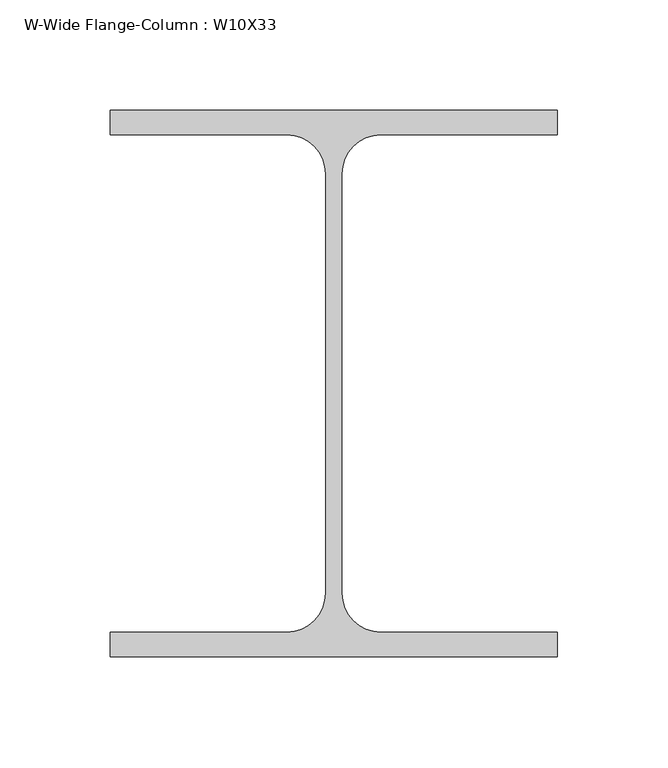
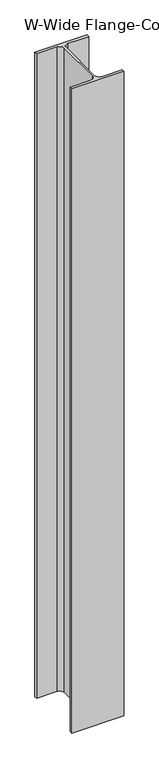
"""IFC4 building model written with IfcOpenShell, lengths in millimetres: column geometry, W-Wide Flange-Column : W10X33."""

import ifcopenshell
import ifcopenshell.guid

model = None  # the IFC model being written
_history = None  # IfcOwnerHistory: only IFC2X3 demands one
_inside = {}  # id of a spatial element -> (the spatial element, [elements in it])
_under = {}  # id of a project, library or spatial element -> (it, [spatial elements below it])
_declared = {}  # id of a project -> (the project, [libraries it declares])
_typed = {}  # id of a type object -> (the type object, [elements of that type])
_made_of = {}  # id of a material, layer set ... -> (it, [elements and type objects made of it])


def new_model(schema):
    """Start an empty IFC model of exactly this schema.

    Asked for "IFC4X3", IfcOpenShell would pick the latest addendum, in which some entities
    have other attributes; the version numbers below select the first issue.
    IFC2X3 requires an IfcOwnerHistory on every rooted entity: one is made here for all.
    """
    global model, _history
    if schema == "IFC4X3":
        model = ifcopenshell.file(schema_version=(4, 3, 0, 0))
    else:
        model = ifcopenshell.file(schema=schema)
    _inside.clear()
    _under.clear()
    _declared.clear()
    _typed.clear()
    _made_of.clear()
    _history = None
    if model.schema == "IFC2X3":
        org = make("IfcOrganization", Name="unknown")
        user = make(
            "IfcPersonAndOrganization",
            ThePerson=make("IfcPerson", FamilyName="unknown"),
            TheOrganization=org,
        )
        app = make(
            "IfcApplication",
            ApplicationDeveloper=org,
            Version="unknown",
            ApplicationFullName="unknown",
            ApplicationIdentifier="unknown",
        )
        _history = make(
            "IfcOwnerHistory",
            OwningUser=user,
            OwningApplication=app,
            ChangeAction="ADDED",
            CreationDate=0,
        )
    return model


def make(cls, **values):
    """One entity of the class cls with the attributes given. An attribute that is None is left unset."""
    return model.create_entity(
        cls, **{name: value for name, value in values.items() if value is not None}
    )


def rooted(cls, **values):
    """An entity with a GlobalId (a new one), such as an element, a storey or a relation."""
    return make(cls, GlobalId=ifcopenshell.guid.new(), OwnerHistory=_history, **values)


def si_unit(unit_type, name, prefix=None):
    """IfcSIUnit, for example si_unit("LENGTHUNIT", "METRE", prefix="MILLI")."""
    return make("IfcSIUnit", UnitType=unit_type, Prefix=prefix, Name=name)


def assignment(units):
    """IfcUnitAssignment: the units of a project."""
    return None if units is None else make("IfcUnitAssignment", Units=units)


def point(xyz):
    """IfcCartesianPoint."""
    return None if xyz is None else make("IfcCartesianPoint", Coordinates=xyz)


def direction(xyz):
    """IfcDirection."""
    return None if xyz is None else make("IfcDirection", DirectionRatios=xyz)


def frame(location, z_axis=None, x_axis=None):
    """IfcAxis2Placement3D, a coordinate frame: its origin and axes. An axis left out is left unset."""
    return make(
        "IfcAxis2Placement3D",
        Location=point(location),
        Axis=direction(z_axis),
        RefDirection=direction(x_axis),
    )


def frame_2d(location, x_axis=None):
    """IfcAxis2Placement2D, a coordinate frame in the plane: its origin and x axis."""
    return make(
        "IfcAxis2Placement2D", Location=point(location), RefDirection=direction(x_axis)
    )


def origin():
    """The frame at (0, 0, 0) with its axes left unset."""
    return frame((0.0, 0.0, 0.0))


def place(relative_to, where):
    """IfcLocalPlacement: puts the frame where relative to a parent placement (None: the world)."""
    return make(
        "IfcLocalPlacement", PlacementRelTo=relative_to, RelativePlacement=where
    )


def context(
    kind, dimensions, precision=None, world=None, true_north=None, identifier=None
):
    """IfcGeometricRepresentationContext, for example the 3D "Model" context."""
    return make(
        "IfcGeometricRepresentationContext",
        ContextIdentifier=identifier,
        ContextType=kind,
        CoordinateSpaceDimension=dimensions,
        Precision=precision,
        WorldCoordinateSystem=world,
        TrueNorth=true_north,
    )


def project(units=None, contexts=None):
    """IfcProject with its units and contexts."""
    return rooted(
        "IfcProject",
        Name="project",
        RepresentationContexts=contexts,
        UnitsInContext=assignment(units),
    )


def spatial(cls, under=None, at=None, **own):
    """A site, building, storey or space (cls), placed at a placement, below another one or the project."""
    s = rooted(cls, ObjectPlacement=at, **own)
    if under is not None:
        _under.setdefault(under.id(), (under, []))[1].append(s)
    return s


def polyline(points):
    """IfcPolyline through the points."""
    return make("IfcPolyline", Points=[point(p) for p in points])


def circle_curve(where, radius):
    """IfcCircle in the frame where."""
    return make("IfcCircle", Position=where, Radius=radius)


def trimmed(basis, trim1, trim2, sense, master):
    """IfcTrimmedCurve: the piece of a basis curve between two trims."""
    return make(
        "IfcTrimmedCurve",
        BasisCurve=basis,
        Trim1=trim1,
        Trim2=trim2,
        SenseAgreement=sense,
        MasterRepresentation=master,
    )


def segment(curve, same_sense, transition):
    """IfcCompositeCurveSegment."""
    return make(
        "IfcCompositeCurveSegment",
        Transition=transition,
        SameSense=same_sense,
        ParentCurve=curve,
    )


def composite_curve(segments, self_intersect=None):
    """IfcCompositeCurve: segments joined end to end."""
    return make("IfcCompositeCurve", Segments=segments, SelfIntersect=self_intersect)


def outline(outer, holes=None, kind="AREA"):
    """IfcArbitraryClosedProfileDef: a profile drawn as a closed curve; with holes, ...WithVoids."""
    if holes is None:
        return make("IfcArbitraryClosedProfileDef", ProfileType=kind, OuterCurve=outer)
    return make(
        "IfcArbitraryProfileDefWithVoids",
        ProfileType=kind,
        OuterCurve=outer,
        InnerCurves=holes,
    )


def extrude(swept, where, along, depth):
    """IfcExtrudedAreaSolid: the profile swept, set in the frame where, extruded along a direction by depth."""
    return make(
        "IfcExtrudedAreaSolid",
        SweptArea=swept,
        Position=where,
        ExtrudedDirection=direction(along),
        Depth=depth,
    )


def shape(context_of_items, identifier, shape_type, items):
    """IfcShapeRepresentation: the items that make up one representation, for example the "Body"."""
    return make(
        "IfcShapeRepresentation",
        ContextOfItems=context_of_items,
        RepresentationIdentifier=identifier,
        RepresentationType=shape_type,
        Items=items,
    )


def source(mapping_origin, context_of_items, identifier, shape_type, items):
    """IfcRepresentationMap: a shape defined once, which mapped items show again and again."""
    return make(
        "IfcRepresentationMap",
        MappingOrigin=mapping_origin,
        MappedRepresentation=shape(context_of_items, identifier, shape_type, items),
    )


def transform(
    local_origin,
    x_axis=None,
    y_axis=None,
    z_axis=None,
    scale=None,
    scale2=None,
    scale3=None,
    uniform=True,
):
    """IfcCartesianTransformationOperator3D, or its non-uniform kind. x_axis, y_axis, z_axis: its Axis1, 2, 3."""
    if uniform:
        return make(
            "IfcCartesianTransformationOperator3D",
            Axis1=direction(x_axis),
            Axis2=direction(y_axis),
            LocalOrigin=point(local_origin),
            Scale=scale,
            Axis3=direction(z_axis),
        )
    return make(
        "IfcCartesianTransformationOperator3DnonUniform",
        Axis1=direction(x_axis),
        Axis2=direction(y_axis),
        LocalOrigin=point(local_origin),
        Scale=scale,
        Axis3=direction(z_axis),
        Scale2=scale2,
        Scale3=scale3,
    )


def mapped(mapping_source, mapping_target):
    """IfcMappedItem: shows the shape of a source again, moved by a transform."""
    return make(
        "IfcMappedItem", MappingSource=mapping_source, MappingTarget=mapping_target
    )


def made_of(thing, what):
    """Note that an element or type object is made of a material, layer set ...; save() writes the relation."""
    if what is not None:
        _made_of.setdefault(what.id(), (what, []))[1].append(thing)
    return thing


def element(
    cls,
    number,
    at=None,
    inside=None,
    cuts=None,
    type_object=None,
    material=None,
    context=None,
    identifier="Body",
    shape_type=None,
    held_by="IfcProductDefinitionShape",
    body=None,
    shapes=None,
    **own,
):
    """One element of the class cls, such as IfcWall. Its Tag is "e" and its number.

    at: its placement. inside: the storey or other place that contains it. cuts: it is an
    opening in that element (IfcRelVoidsElement). A single representation is given by context,
    identifier, shape_type and body (its items); several are given by shapes. held_by: the class
    of the entity that holds the representations. save() writes the other relations.
    """
    e = rooted(cls, Tag="e%d" % number, ObjectPlacement=at, **own)
    if body is not None:
        shapes = [shape(context, identifier, shape_type, body)]
    if shapes is not None:
        e.Representation = make(held_by, Representations=shapes)
    if inside is not None:
        _inside.setdefault(inside.id(), (inside, []))[1].append(e)
    if cuts is not None:
        rooted(
            "IfcRelVoidsElement", RelatingBuildingElement=cuts, RelatedOpeningElement=e
        )
    if type_object is not None:
        _typed.setdefault(type_object.id(), (type_object, []))[1].append(e)
    return made_of(e, material)


def aggregate(whole, parts):
    """IfcRelAggregates: a whole, such as a stair, and the parts it consists of."""
    return rooted("IfcRelAggregates", RelatingObject=whole, RelatedObjects=parts)


def save(model, path):
    """Write the relations noted so far, then the file.

    IfcRelAggregates (storeys below a building ...), IfcRelContainedInSpatialStructure (elements
    in a storey), IfcRelDefinesByType, IfcRelAssociatesMaterial and IfcRelDeclares: one each for
    every whole, place, type object, material and project.
    """
    for whole, parts in _under.values():
        aggregate(whole, parts)
    for where, things in _inside.values():
        rooted(
            "IfcRelContainedInSpatialStructure",
            RelatedElements=things,
            RelatingStructure=where,
        )
    for kind, things in _typed.values():
        rooted("IfcRelDefinesByType", RelatedObjects=things, RelatingType=kind)
    for what, things in _made_of.values():
        rooted("IfcRelAssociatesMaterial", RelatedObjects=things, RelatingMaterial=what)
    for by, libraries in _declared.values():
        rooted("IfcRelDeclares", RelatingContext=by, RelatedDefinitions=libraries)
    model.write(path)


def w_wide_flange_column_w10x33_651e5602(model_context):
    return source(origin(), model_context, "Body", "SweptSolid", [
        extrude(outline(composite_curve([segment(polyline([(101.092, 123.571), (101.092, 112.522), (21.209, 112.522)]), True, "CONTINUOUS"), segment(trimmed(circle_curve(frame_2d((21.209, 94.996)), 17.526), [point((21.209, 112.522))], [point((3.683, 94.996))], True, "CARTESIAN"), True, "CONTINUOUS"), segment(polyline([(3.683, 94.996), (3.683, -94.996)]), True, "CONTINUOUS"), segment(trimmed(circle_curve(frame_2d((21.209, -94.996)), 17.526), [point((3.683, -94.996))], [point((21.209, -112.522))], True, "CARTESIAN"), True, "CONTINUOUS"), segment(polyline([(21.209, -112.522), (101.092, -112.522), (101.092, -123.571), (-101.092, -123.571), (-101.092, -112.522), (-21.209, -112.522)]), True, "CONTINUOUS"), segment(trimmed(circle_curve(frame_2d((-21.209, -94.996)), 17.526), [point((-21.209, -112.522))], [point((-3.683, -94.996))], True, "CARTESIAN"), True, "CONTINUOUS"), segment(polyline([(-3.683, -94.996), (-3.683, 94.996)]), True, "CONTINUOUS"), segment(trimmed(circle_curve(frame_2d((-21.209, 94.996)), 17.526), [point((-3.683, 94.996))], [point((-21.209, 112.522))], True, "CARTESIAN"), True, "CONTINUOUS"), segment(polyline([(-21.209, 112.522), (-101.092, 112.522), (-101.092, 123.571), (101.092, 123.571)]), True, "CONTINUOUS")], self_intersect=False)), frame((0.0, 0.0, 19253.2), z_axis=(0.0, 0.0, 1.0), x_axis=(1.0, 0.0, 0.0)), (0.0, 0.0, 1.0), 2641.6),
    ])


if __name__ == "__main__":
    model = new_model("IFC4")
    model_context = context("Model", 3, world=origin())
    ifc_project = project(units=[si_unit("LENGTHUNIT", "METRE", prefix="MILLI")], contexts=[model_context])
    site = spatial("IfcSite", under=ifc_project)
    building = spatial("IfcBuilding", under=site)
    placement = place(None, origin())
    w_wide_flange_column_w10x33_shape = w_wide_flange_column_w10x33_651e5602(model_context)
    element("IfcColumn", 1, ObjectType="W-Wide Flange-Column : W10X33", at=placement, inside=building, context=model_context, shape_type="MappedRepresentation", body=[
        mapped(w_wide_flange_column_w10x33_shape, transform((0.0, 0.0, 0.0), x_axis=(1.0, 0.0, 0.0), y_axis=(0.0, 1.0, 0.0), z_axis=(0.0, 0.0, 1.0))),
    ])
    save(model, "model.ifc")

# Revit data of these elements
# Type "W-Wide Flange-Column : W10X33"
#   Assembly Code = "B10"
#   W = 33
#   bf = 0' - 7.96"
#   d = 0' - 9.73"
#   k = 0' - 1 1/8"
#   kr = 0' - 0.69"
#   tf = 0' - 0.435"
#   tw = 0' - 0.29"
#   A = 0.0674306 SF
#   Structural Material [instance default] = Steel ASTM A992
# Element 1 (IfcColumn, "W-Wide Flange-Column : W10X33")
#   Materials on its faces: "Steel ASTM A992"
# Materials
#   "Steel ASTM A992": class "Metal", colour RGB 199 199 199, transparency 0, Description = "Structural steel 50ksi", Cost = 0
